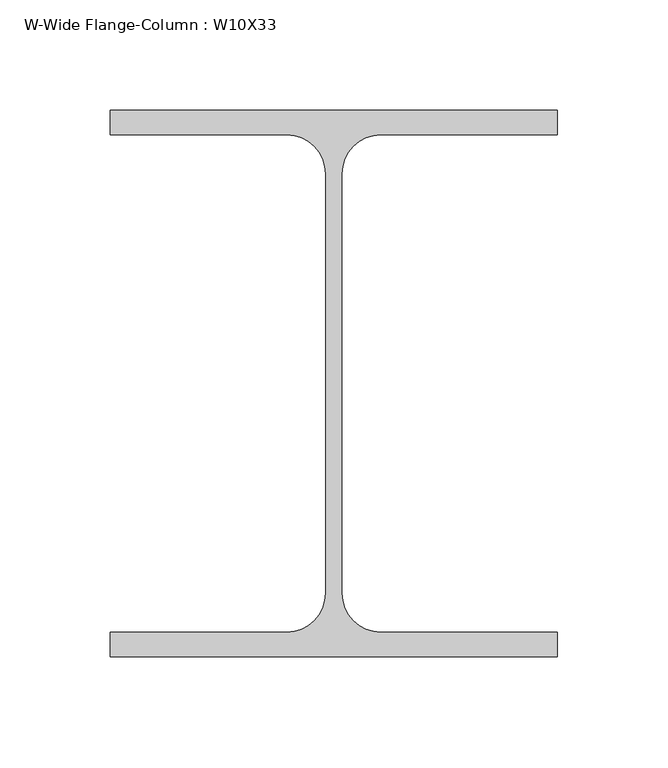
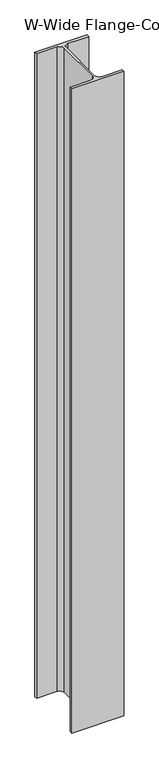
"""IFC4 building model written with IfcOpenShell, lengths in millimetres: column geometry, W-Wide Flange-Column : W10X33."""

from ifc_helpers import new_model, si_unit, point, frame, frame_2d, origin, place, context, project, spatial, polyline, circle_curve, trimmed, segment, composite_curve, outline, extrude, source, transform, mapped, element, save


def w_wide_flange_column_w10x33_651e5602(model_context):
    return source(origin(), model_context, "Body", "SweptSolid", [
        extrude(outline(composite_curve([segment(polyline([(101.092, 123.571), (101.092, 112.522), (21.209, 112.522)]), True, "CONTINUOUS"), segment(trimmed(circle_curve(frame_2d((21.209, 94.996)), 17.526), [point((21.209, 112.522))], [point((3.683, 94.996))], True, "CARTESIAN"), True, "CONTINUOUS"), segment(polyline([(3.683, 94.996), (3.683, -94.996)]), True, "CONTINUOUS"), segment(trimmed(circle_curve(frame_2d((21.209, -94.996)), 17.526), [point((3.683, -94.996))], [point((21.209, -112.522))], True, "CARTESIAN"), True, "CONTINUOUS"), segment(polyline([(21.209, -112.522), (101.092, -112.522), (101.092, -123.571), (-101.092, -123.571), (-101.092, -112.522), (-21.209, -112.522)]), True, "CONTINUOUS"), segment(trimmed(circle_curve(frame_2d((-21.209, -94.996)), 17.526), [point((-21.209, -112.522))], [point((-3.683, -94.996))], True, "CARTESIAN"), True, "CONTINUOUS"), segment(polyline([(-3.683, -94.996), (-3.683, 94.996)]), True, "CONTINUOUS"), segment(trimmed(circle_curve(frame_2d((-21.209, 94.996)), 17.526), [point((-3.683, 94.996))], [point((-21.209, 112.522))], True, "CARTESIAN"), True, "CONTINUOUS"), segment(polyline([(-21.209, 112.522), (-101.092, 112.522), (-101.092, 123.571), (101.092, 123.571)]), True, "CONTINUOUS")], self_intersect=False)), frame((0.0, 0.0, 19253.2), z_axis=(0.0, 0.0, 1.0), x_axis=(1.0, 0.0, 0.0)), (0.0, 0.0, 1.0), 2641.6),
    ])


if __name__ == "__main__":
    model = new_model("IFC4")
    model_context = context("Model", 3, world=origin())
    ifc_project = project(units=[si_unit("LENGTHUNIT", "METRE", prefix="MILLI")], contexts=[model_context])
    site = spatial("IfcSite", under=ifc_project)
    building = spatial("IfcBuilding", under=site)
    placement = place(None, origin())
    w_wide_flange_column_w10x33_shape = w_wide_flange_column_w10x33_651e5602(model_context)
    element("IfcColumn", 1, ObjectType="W-Wide Flange-Column : W10X33", at=placement, inside=building, context=model_context, shape_type="MappedRepresentation", body=[
        mapped(w_wide_flange_column_w10x33_shape, transform((0.0, 0.0, 0.0), x_axis=(1.0, 0.0, 0.0), y_axis=(0.0, 1.0, 0.0), z_axis=(0.0, 0.0, 1.0))),
    ])
    save(model, "model.ifc")

# Revit data of these elements
# Type "W-Wide Flange-Column : W10X33"
#   Assembly Code = "B10"
#   W = 33
#   bf = 0' - 7.96"
#   d = 0' - 9.73"
#   k = 0' - 1 1/8"
#   kr = 0' - 0.69"
#   tf = 0' - 0.435"
#   tw = 0' - 0.29"
#   A = 0.0674306 SF
#   Structural Material [instance default] = Steel ASTM A992
# Element 1 (IfcColumn, "W-Wide Flange-Column : W10X33")
#   Materials on its faces: "Steel ASTM A992"
# Materials
#   "Steel ASTM A992": class "Metal", colour RGB 199 199 199, transparency 0, Description = "Structural steel 50ksi", Cost = 0
